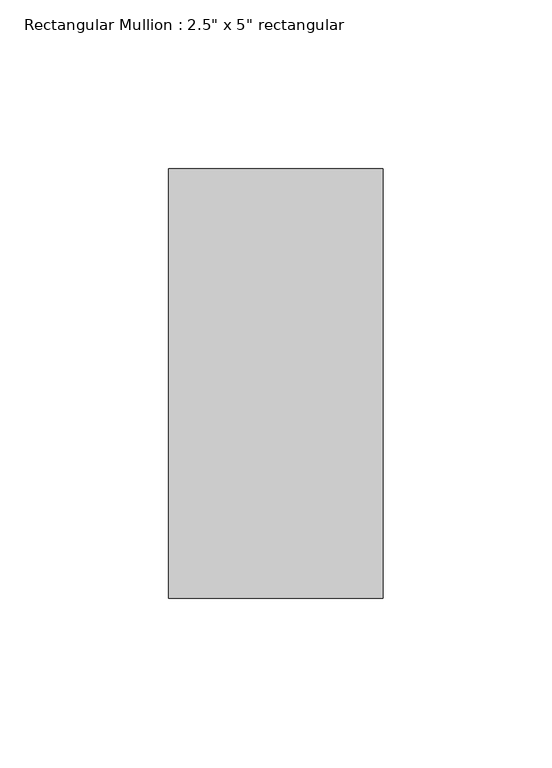
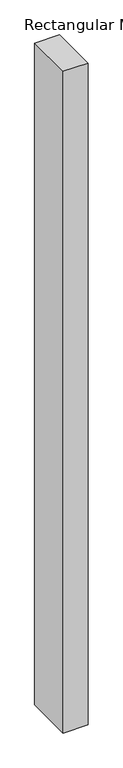
"""IFC4 building model written with IfcOpenShell, lengths in millimetres: member geometry."""

from ifc_helpers import new_model, si_unit, frame, origin, place, context, project, spatial, polyline, outline, extrude, source, transform, mapped, element, save


def member_c3fe432b(model_context):
    return source(origin(), model_context, "Body", "SweptSolid", [
        extrude(outline(polyline([(31.75, 63.5), (31.75, -63.5), (-31.75, -63.5), (-31.75, 63.5), (31.75, 63.5)])), frame((0.0, 0.0, -1797.05), z_axis=(0.0, 0.0, 1.0), x_axis=(1.0, 0.0, 0.0)), (0.0, 0.0, 1.0), 1797.05),
    ])


if __name__ == "__main__":
    model = new_model("IFC4")
    model_context = context("Model", 3, world=origin())
    ifc_project = project(units=[si_unit("LENGTHUNIT", "METRE", prefix="MILLI")], contexts=[model_context])
    site = spatial("IfcSite", under=ifc_project)
    building = spatial("IfcBuilding", under=site)
    placement = place(None, origin())
    member_shape = member_c3fe432b(model_context)
    element("IfcMember", 1, ObjectType="Rectangular Mullion : 2.5\" x 5\" rectangular", at=placement, inside=building, context=model_context, shape_type="MappedRepresentation", body=[
        mapped(member_shape, transform((0.0, 0.0, 0.0), x_axis=(1.0, 0.0, 0.0), y_axis=(0.0, 1.0, 0.0), z_axis=(0.0, 0.0, 1.0))),
    ])
    save(model, "model.ifc")

# Revit data of these elements
# Type "Rectangular Mullion : 2.5\" x 5\" rectangular"
#   built-in parameter 1007304 = 0.416667 (stored number, unit not read)
#   built-in parameter 1007301 = 0.104167 (stored number, unit not read)
#   built-in parameter 1007300 = 0.104167 (stored number, unit not read)
# Element 1 (IfcMember, "Rectangular Mullion : 2.5\" x 5\" rectangular")
#   Materials on its faces: "Aluminum"
# Materials
#   "Aluminum": class "Metal", colour RGB 247 247 247, transparency 0, Description = "Aluminum 6061", Cost = 0
